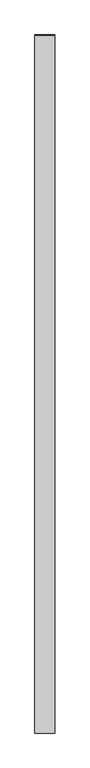
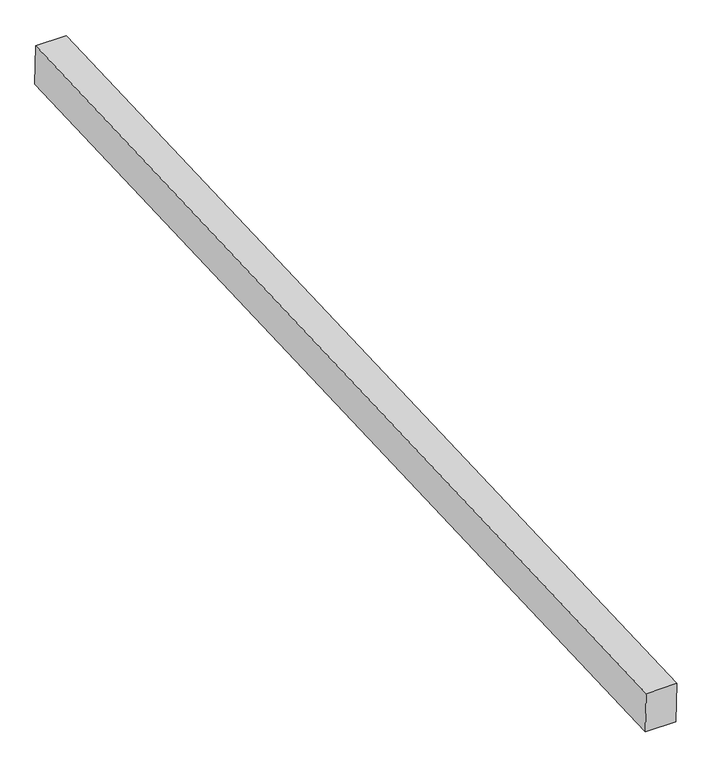
"""IFC4 building model written with IfcOpenShell, lengths in millimetres: proxy geometry, Generic Models 7:Generic Models 1:8:Generic Models 1:8 : Generic Models 7:Generic Models 1:337419:43 : Generic Models 7:Generic Models 1:8:Generic Models 1:8 : Generic Models 7:Generic Models 1:337419:315935."""

from ifc_helpers import new_model, si_unit, frame, origin, place, context, project, spatial, polyline, outline, extrude, source, transform, mapped, element, save


def generic_models_4ec61bfd(model_context):
    return source(origin(), model_context, "Body", "SweptSolid", [
        extrude(outline(polyline([(-581229.2495411, 3818.908703), (-576356.3266468, 4021.9471569), (-576348.7597251, 3831.5971524), (-581221.3189223, 3628.5738526), (-581229.2495411, 3818.908703)])), frame((661070.3117239, 0.0, 0.0), z_axis=(1.0, 0.0, 0.0), x_axis=(0.0, 1.0, 0.0)), (0.0, 0.0, 1.0), 139.7),
    ])


if __name__ == "__main__":
    model = new_model("IFC4")
    model_context = context("Model", 3, world=origin())
    ifc_project = project(units=[si_unit("LENGTHUNIT", "METRE", prefix="MILLI")], contexts=[model_context])
    site = spatial("IfcSite", under=ifc_project)
    building = spatial("IfcBuilding", under=site)
    placement = place(None, origin())
    generic_models_shape = generic_models_4ec61bfd(model_context)
    element("IfcBuildingElementProxy", 1, Name="Generic Models 7:Generic Models 1:8:Generic Models 1:8 : Generic Models 7:Generic Models 1:337419:43 : Generic Models 7:Generic Models 1:8:Generic Models 1:8 : Generic Models 7:Generic Models 1:337419:315935", ObjectType="Generic Models 7:Generic Models 1:8:Generic Models 1:8 : Generic Models 7:Generic Models 1:337419:43 : Generic Models 7:Generic Models 1:8:Generic Models 1:8 : Generic Models 7:Generic Models 1:337419:315935", at=placement, inside=building, context=model_context, shape_type="MappedRepresentation", body=[
        mapped(generic_models_shape, transform((0.0, 0.0, 0.0), x_axis=(1.0, 0.0, 0.0), y_axis=(0.0, 1.0, 0.0), z_axis=(0.0, 0.0, 1.0))),
    ])
    save(model, "model.ifc")

# Revit data of these elements
# Type "Generic Models 7:Generic Models 1:8:Generic Models 1:8 : Generic Models 7:Generic Models 1:337419:43 : Generic Models 7:Generic Models 1:8:Generic Models 1:8 : Generic Models 7:Generic Models 1:337419:315935"
#   NameOverride = "Generic Models 7:Generic Models 1:8:Generic Models 1:8 : Generic Models 7:Generic Models 1:337419:315935"
#   ObjectTypeOverride = "Generic Models 1:8 : Generic Models 7:Generic Models 1:337419"
#   Reference = "Generic Models 1"
#   Tag = "315935"
# Element 1 (IfcBuildingElementProxy, "Generic Models 7:Generic Models 1:8:Generic Models 1:8 : Generic Models 7:Generic Models 1:337419:43 : Generic Models 7:Generic Models 1:8:Generic Models 1:8 : Generic Models 7:Generic Models 1:337419:315935")
#   Materials on its faces: "5 1/2\" X 7 1/2\" EXTERIOR GRADE GLULAM BEAMS"
# Materials
#   "5 1/2\" X 7 1/2\" EXTERIOR GRADE GLULAM BEAMS": class "Wood", colour RGB 183 134 68, transparency 0, Keynote = "M06181300.01", Description = "Pinus Echinata", Cost = 0
